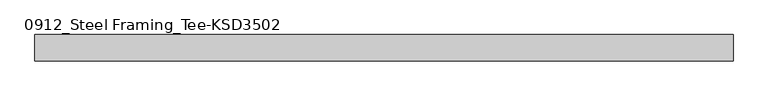
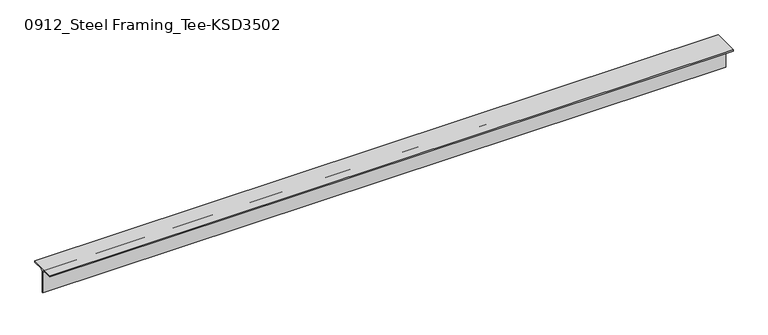
"""IFC4 building model written with IfcOpenShell, lengths in millimetres: member geometry, 0912_Steel Framing_Tee-KSD3502 : H_SB_ASB_CT-150x150x6.5x9."""

from ifc_helpers import new_model, si_unit, point, frame, frame_2d, origin, place, context, project, spatial, polyline, circle_curve, trimmed, segment, composite_curve, outline, extrude, source, transform, mapped, element, save


def member_0912_steel_framing_tee_ksd3502_72b9a402(model_context):
    return source(origin(), model_context, "Body", "SweptSolid", [
        extrude(outline(composite_curve([segment(polyline([(-75.0, 75.0), (75.0, 75.0), (75.0, 66.0), (16.25, 66.0)]), True, "CONTINUOUS"), segment(trimmed(circle_curve(frame_2d((16.25, 53.0)), 13.0), [point((16.25, 66.0))], [point((3.25, 53.0))], True, "CARTESIAN"), True, "CONTINUOUS"), segment(polyline([(3.25, 53.0), (3.25, -75.0), (-3.25, -75.0), (-3.25, 53.0)]), True, "CONTINUOUS"), segment(trimmed(circle_curve(frame_2d((-16.25, 53.0)), 13.0), [point((-3.25, 53.0))], [point((-16.25, 66.0))], True, "CARTESIAN"), True, "CONTINUOUS"), segment(polyline([(-16.25, 66.0), (-75.0, 66.0), (-75.0, 75.0)]), True, "CONTINUOUS")], self_intersect=False)), frame((-1979.35, 0.0, 0.0), z_axis=(1.0, 0.0, 0.0), x_axis=(0.0, 1.0, 0.0)), (0.0, 0.0, 1.0), 3955.0),
    ])


if __name__ == "__main__":
    model = new_model("IFC4")
    model_context = context("Model", 3, world=origin())
    ifc_project = project(units=[si_unit("LENGTHUNIT", "METRE", prefix="MILLI")], contexts=[model_context])
    site = spatial("IfcSite", under=ifc_project)
    building = spatial("IfcBuilding", under=site)
    placement = place(None, origin())
    member_0912_steel_framing_tee_ksd3502_shape = member_0912_steel_framing_tee_ksd3502_72b9a402(model_context)
    element("IfcMember", 1, ObjectType="0912_Steel Framing_Tee-KSD3502 : H_SB_ASB_CT-150x150x6.5x9", at=placement, inside=building, context=model_context, shape_type="MappedRepresentation", body=[
        mapped(member_0912_steel_framing_tee_ksd3502_shape, transform((0.0, 0.0, 0.0), x_axis=(1.0, 0.0, 0.0), y_axis=(0.0, 1.0, 0.0), z_axis=(0.0, 0.0, 1.0))),
    ])
    save(model, "model.ifc")

# Revit data of these elements
# Type "0912_Steel Framing_Tee-KSD3502 : H_SB_ASB_CT-150x150x6.5x9"
#   H_WM Code_1 = "S01AA003-00001 | Main Steel Structure Fabrication Work | Shelter/Building | Light Steel - Standard (30KG/M>Weight) | Material: (   )"
#   H_WM Code_2 = "S03AA029-00001 | Main Steel Structure Erection Work | Shelter/Building | Light Steel (30KG/M>Weight) | Material: (   )"
#   H_WM Code_3 = "S01AA010-00001 | Main Steel Structure Fabrication Work | Shelter/Building | Steel Painting/Coating | for Non-Fireproofed Steel Surface, Surface Preparation, Primer, Second & Final Coat | Material: (   )"
#   H_Q'ty Cal Type Tag = "SB-Q2"
#   Width = 15.0 cm
#   Web Thickness = 0.65 cm
#   Web Fillet = 1.3 cm
#   Section Area = 23.39 cm²
#   Perimeter = 0.60 m²/m
#   Nominal Weight = 18.40 kgf/m
#   Height = 15.0 cm
#   Flange Thickness = 0.9 cm
#   Centroid Vertical = 7.5 cm
#   Centroid Horizontal = 7.5 cm
#   Length [instance default] = 1.5000 m
#   Structural Material [instance default] = Steel, 45-345
#   Warping Constant = (empty or 0)
#   Torsional Moment of Inertia = 0
#   Section Name Key = ""
#   Plastic Modulus weak axis = 0
#   Plastic Modulus strong axis = 0
#   Moment of Inertia weak axis = 0
#   Moment of Inertia strong axis = 0
#   Elastic Modulus weak axis = 0
#   Elastic Modulus strong axis = 0
#   Bolt Spacing = 0
#   Assembly Code = ""
# Element 1 (IfcMember, "0912_Steel Framing_Tee-KSD3502 : H_SB_ASB_CT-150x150x6.5x9")
#   Structural Material = none
# Materials
#   "Steel, 45-345": class "Metal", colour RGB 189 187 185, transparency 0, Description = "Steel 345 MPa", Cost = 0
